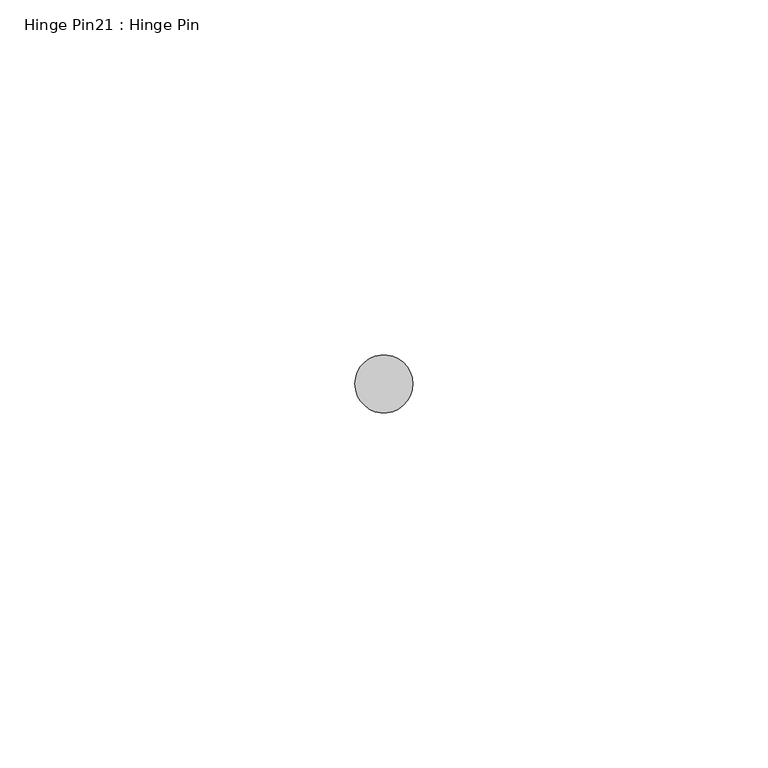
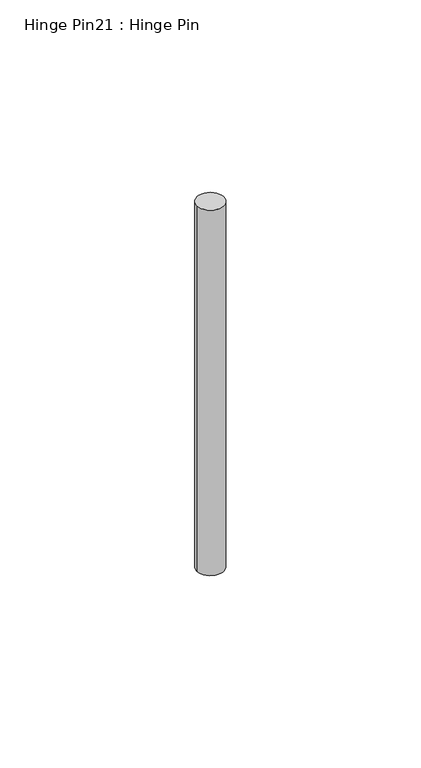
"""IFC4 building model written with IfcOpenShell, lengths in millimetres: proxy geometry, Hinge Pin21 : Hinge Pin."""

from ifc_helpers import new_model, si_unit, point, frame, frame_2d, origin, place, context, project, spatial, circle_curve, trimmed, segment, composite_curve, outline, extrude, source, transform, mapped, element, save


def hinge_pin21_hinge_pin_7a47ebab(model_context):
    return source(origin(), model_context, "Body", "SweptSolid", [
        extrude(outline(composite_curve([segment(trimmed(circle_curve(frame_2d((587319.1320739, -536310.3652841)), 4.0894), [point((587315.0426739, -536310.3652841))], [point((587323.2214739, -536310.3652841))], False, "CARTESIAN"), True, "CONTINUOUS"), segment(trimmed(circle_curve(frame_2d((587319.1320739, -536310.3652841)), 4.0894), [point((587323.2214739, -536310.3652841))], [point((587315.0426739, -536310.3652841))], False, "CARTESIAN"), True, "CONTINUOUS")], self_intersect=False)), frame((0.0, 0.0, 315.7140625), z_axis=(0.0, 0.0, 1.0), x_axis=(1.0, 0.0, 0.0)), (0.0, 0.0, 1.0), 117.871875),
    ])


if __name__ == "__main__":
    model = new_model("IFC4")
    model_context = context("Model", 3, world=origin())
    ifc_project = project(units=[si_unit("LENGTHUNIT", "METRE", prefix="MILLI")], contexts=[model_context])
    site = spatial("IfcSite", under=ifc_project)
    building = spatial("IfcBuilding", under=site)
    placement = place(None, origin())
    hinge_pin21_hinge_pin_shape = hinge_pin21_hinge_pin_7a47ebab(model_context)
    element("IfcBuildingElementProxy", 1, Name="Hinge Pin21 : Hinge Pin", ObjectType="Hinge Pin21 : Hinge Pin", at=placement, inside=building, context=model_context, shape_type="MappedRepresentation", body=[
        mapped(hinge_pin21_hinge_pin_shape, transform((0.0, 0.0, 0.0), x_axis=(1.0, 0.0, 0.0), y_axis=(0.0, 1.0, 0.0), z_axis=(0.0, 0.0, 1.0))),
    ])
    save(model, "model.ifc")

# Revit data of these elements
# Element 1 (IfcBuildingElementProxy, "Hinge Pin21 : Hinge Pin")
#   Materials on its faces: "6\"X6\" WELD-ON STL BUTT HINGE"
# Materials
#   "6\"X6\" WELD-ON STL BUTT HINGE": class "Metal", colour RGB 189 187 185, transparency 0, Description = "Carbon steel", Cost = 0
